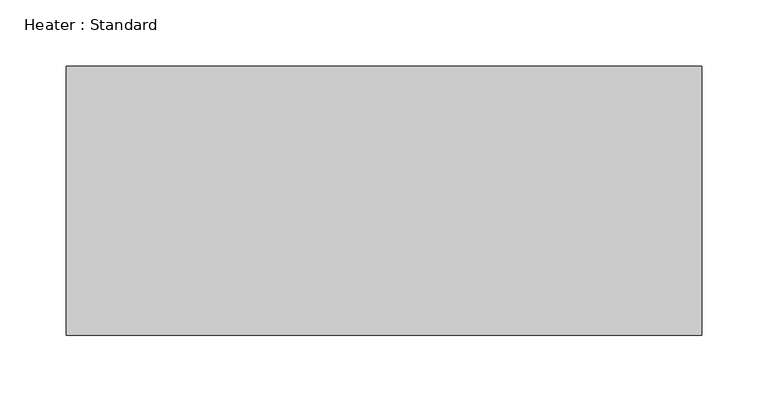
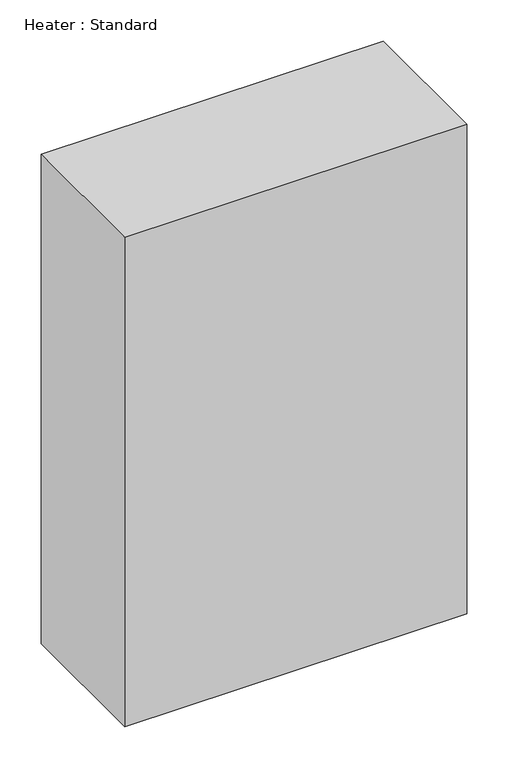
"""IFC4 building model written with IfcOpenShell, lengths in millimetres: proxy geometry, Heater : Standard."""

import ifcopenshell
import ifcopenshell.guid

model = None  # the IFC model being written
_history = None  # IfcOwnerHistory: only IFC2X3 demands one
_inside = {}  # id of a spatial element -> (the spatial element, [elements in it])
_under = {}  # id of a project, library or spatial element -> (it, [spatial elements below it])
_declared = {}  # id of a project -> (the project, [libraries it declares])
_typed = {}  # id of a type object -> (the type object, [elements of that type])
_made_of = {}  # id of a material, layer set ... -> (it, [elements and type objects made of it])


def new_model(schema):
    """Start an empty IFC model of exactly this schema.

    Asked for "IFC4X3", IfcOpenShell would pick the latest addendum, in which some entities
    have other attributes; the version numbers below select the first issue.
    IFC2X3 requires an IfcOwnerHistory on every rooted entity: one is made here for all.
    """
    global model, _history
    if schema == "IFC4X3":
        model = ifcopenshell.file(schema_version=(4, 3, 0, 0))
    else:
        model = ifcopenshell.file(schema=schema)
    _inside.clear()
    _under.clear()
    _declared.clear()
    _typed.clear()
    _made_of.clear()
    _history = None
    if model.schema == "IFC2X3":
        org = make("IfcOrganization", Name="unknown")
        user = make(
            "IfcPersonAndOrganization",
            ThePerson=make("IfcPerson", FamilyName="unknown"),
            TheOrganization=org,
        )
        app = make(
            "IfcApplication",
            ApplicationDeveloper=org,
            Version="unknown",
            ApplicationFullName="unknown",
            ApplicationIdentifier="unknown",
        )
        _history = make(
            "IfcOwnerHistory",
            OwningUser=user,
            OwningApplication=app,
            ChangeAction="ADDED",
            CreationDate=0,
        )
    return model


def make(cls, **values):
    """One entity of the class cls with the attributes given. An attribute that is None is left unset."""
    return model.create_entity(
        cls, **{name: value for name, value in values.items() if value is not None}
    )


def rooted(cls, **values):
    """An entity with a GlobalId (a new one), such as an element, a storey or a relation."""
    return make(cls, GlobalId=ifcopenshell.guid.new(), OwnerHistory=_history, **values)


def si_unit(unit_type, name, prefix=None):
    """IfcSIUnit, for example si_unit("LENGTHUNIT", "METRE", prefix="MILLI")."""
    return make("IfcSIUnit", UnitType=unit_type, Prefix=prefix, Name=name)


def assignment(units):
    """IfcUnitAssignment: the units of a project."""
    return None if units is None else make("IfcUnitAssignment", Units=units)


def point(xyz):
    """IfcCartesianPoint."""
    return None if xyz is None else make("IfcCartesianPoint", Coordinates=xyz)


def direction(xyz):
    """IfcDirection."""
    return None if xyz is None else make("IfcDirection", DirectionRatios=xyz)


def frame(location, z_axis=None, x_axis=None):
    """IfcAxis2Placement3D, a coordinate frame: its origin and axes. An axis left out is left unset."""
    return make(
        "IfcAxis2Placement3D",
        Location=point(location),
        Axis=direction(z_axis),
        RefDirection=direction(x_axis),
    )


def origin():
    """The frame at (0, 0, 0) with its axes left unset."""
    return frame((0.0, 0.0, 0.0))


def origin_with_axes():
    """The frame at (0, 0, 0) with the z axis (0, 0, 1) and the x axis (1, 0, 0) written out."""
    return frame((0.0, 0.0, 0.0), z_axis=(0.0, 0.0, 1.0), x_axis=(1.0, 0.0, 0.0))


def place(relative_to, where):
    """IfcLocalPlacement: puts the frame where relative to a parent placement (None: the world)."""
    return make(
        "IfcLocalPlacement", PlacementRelTo=relative_to, RelativePlacement=where
    )


def context(
    kind, dimensions, precision=None, world=None, true_north=None, identifier=None
):
    """IfcGeometricRepresentationContext, for example the 3D "Model" context."""
    return make(
        "IfcGeometricRepresentationContext",
        ContextIdentifier=identifier,
        ContextType=kind,
        CoordinateSpaceDimension=dimensions,
        Precision=precision,
        WorldCoordinateSystem=world,
        TrueNorth=true_north,
    )


def project(units=None, contexts=None):
    """IfcProject with its units and contexts."""
    return rooted(
        "IfcProject",
        Name="project",
        RepresentationContexts=contexts,
        UnitsInContext=assignment(units),
    )


def spatial(cls, under=None, at=None, **own):
    """A site, building, storey or space (cls), placed at a placement, below another one or the project."""
    s = rooted(cls, ObjectPlacement=at, **own)
    if under is not None:
        _under.setdefault(under.id(), (under, []))[1].append(s)
    return s


def polyline(points):
    """IfcPolyline through the points."""
    return make("IfcPolyline", Points=[point(p) for p in points])


def outline(outer, holes=None, kind="AREA"):
    """IfcArbitraryClosedProfileDef: a profile drawn as a closed curve; with holes, ...WithVoids."""
    if holes is None:
        return make("IfcArbitraryClosedProfileDef", ProfileType=kind, OuterCurve=outer)
    return make(
        "IfcArbitraryProfileDefWithVoids",
        ProfileType=kind,
        OuterCurve=outer,
        InnerCurves=holes,
    )


def extrude(swept, where, along, depth):
    """IfcExtrudedAreaSolid: the profile swept, set in the frame where, extruded along a direction by depth."""
    return make(
        "IfcExtrudedAreaSolid",
        SweptArea=swept,
        Position=where,
        ExtrudedDirection=direction(along),
        Depth=depth,
    )


def shape(context_of_items, identifier, shape_type, items):
    """IfcShapeRepresentation: the items that make up one representation, for example the "Body"."""
    return make(
        "IfcShapeRepresentation",
        ContextOfItems=context_of_items,
        RepresentationIdentifier=identifier,
        RepresentationType=shape_type,
        Items=items,
    )


def source(mapping_origin, context_of_items, identifier, shape_type, items):
    """IfcRepresentationMap: a shape defined once, which mapped items show again and again."""
    return make(
        "IfcRepresentationMap",
        MappingOrigin=mapping_origin,
        MappedRepresentation=shape(context_of_items, identifier, shape_type, items),
    )


def transform(
    local_origin,
    x_axis=None,
    y_axis=None,
    z_axis=None,
    scale=None,
    scale2=None,
    scale3=None,
    uniform=True,
):
    """IfcCartesianTransformationOperator3D, or its non-uniform kind. x_axis, y_axis, z_axis: its Axis1, 2, 3."""
    if uniform:
        return make(
            "IfcCartesianTransformationOperator3D",
            Axis1=direction(x_axis),
            Axis2=direction(y_axis),
            LocalOrigin=point(local_origin),
            Scale=scale,
            Axis3=direction(z_axis),
        )
    return make(
        "IfcCartesianTransformationOperator3DnonUniform",
        Axis1=direction(x_axis),
        Axis2=direction(y_axis),
        LocalOrigin=point(local_origin),
        Scale=scale,
        Axis3=direction(z_axis),
        Scale2=scale2,
        Scale3=scale3,
    )


def mapped(mapping_source, mapping_target):
    """IfcMappedItem: shows the shape of a source again, moved by a transform."""
    return make(
        "IfcMappedItem", MappingSource=mapping_source, MappingTarget=mapping_target
    )


def made_of(thing, what):
    """Note that an element or type object is made of a material, layer set ...; save() writes the relation."""
    if what is not None:
        _made_of.setdefault(what.id(), (what, []))[1].append(thing)
    return thing


def element(
    cls,
    number,
    at=None,
    inside=None,
    cuts=None,
    type_object=None,
    material=None,
    context=None,
    identifier="Body",
    shape_type=None,
    held_by="IfcProductDefinitionShape",
    body=None,
    shapes=None,
    **own,
):
    """One element of the class cls, such as IfcWall. Its Tag is "e" and its number.

    at: its placement. inside: the storey or other place that contains it. cuts: it is an
    opening in that element (IfcRelVoidsElement). A single representation is given by context,
    identifier, shape_type and body (its items); several are given by shapes. held_by: the class
    of the entity that holds the representations. save() writes the other relations.
    """
    e = rooted(cls, Tag="e%d" % number, ObjectPlacement=at, **own)
    if body is not None:
        shapes = [shape(context, identifier, shape_type, body)]
    if shapes is not None:
        e.Representation = make(held_by, Representations=shapes)
    if inside is not None:
        _inside.setdefault(inside.id(), (inside, []))[1].append(e)
    if cuts is not None:
        rooted(
            "IfcRelVoidsElement", RelatingBuildingElement=cuts, RelatedOpeningElement=e
        )
    if type_object is not None:
        _typed.setdefault(type_object.id(), (type_object, []))[1].append(e)
    return made_of(e, material)


def aggregate(whole, parts):
    """IfcRelAggregates: a whole, such as a stair, and the parts it consists of."""
    return rooted("IfcRelAggregates", RelatingObject=whole, RelatedObjects=parts)


def save(model, path):
    """Write the relations noted so far, then the file.

    IfcRelAggregates (storeys below a building ...), IfcRelContainedInSpatialStructure (elements
    in a storey), IfcRelDefinesByType, IfcRelAssociatesMaterial and IfcRelDeclares: one each for
    every whole, place, type object, material and project.
    """
    for whole, parts in _under.values():
        aggregate(whole, parts)
    for where, things in _inside.values():
        rooted(
            "IfcRelContainedInSpatialStructure",
            RelatedElements=things,
            RelatingStructure=where,
        )
    for kind, things in _typed.values():
        rooted("IfcRelDefinesByType", RelatedObjects=things, RelatingType=kind)
    for what, things in _made_of.values():
        rooted("IfcRelAssociatesMaterial", RelatedObjects=things, RelatingMaterial=what)
    for by, libraries in _declared.values():
        rooted("IfcRelDeclares", RelatingContext=by, RelatedDefinitions=libraries)
    model.write(path)


def heater_standard_9b13520e(model_context):
    return source(origin(), model_context, "Body", "SweptSolid", [
        extrude(outline(polyline([(240.0101563, 0.0), (240.0101563, -203.2), (-240.0101562, -203.2), (-240.0101562, 0.0), (240.0101563, 0.0)])), origin_with_axes(), (0.0, 0.0, 1.0), 726.4796875),
    ])


if __name__ == "__main__":
    model = new_model("IFC4")
    model_context = context("Model", 3, world=origin())
    ifc_project = project(units=[si_unit("LENGTHUNIT", "METRE", prefix="MILLI")], contexts=[model_context])
    site = spatial("IfcSite", under=ifc_project)
    building = spatial("IfcBuilding", under=site)
    placement = place(None, origin())
    heater_standard_shape = heater_standard_9b13520e(model_context)
    element("IfcBuildingElementProxy", 1, Name="Heater : Standard", ObjectType="Heater : Standard", at=placement, inside=building, context=model_context, shape_type="MappedRepresentation", body=[
        mapped(heater_standard_shape, transform((0.0, 0.0, 0.0), x_axis=(1.0, 0.0, 0.0), y_axis=(0.0, 1.0, 0.0), z_axis=(0.0, 0.0, 1.0))),
    ])
    save(model, "model.ifc")

# Revit data of these elements
# Type "Heater : Standard"
#   Label = "H"
#   Width = 0' - 8"
#   Voltage = 120 V
#   Length = 1' - 6 115/128"
#   Height = 2' - 4 77/128"
#   Apparent Load = 1500 VA
#   Number of Poles = 1
#   Load Classification = Heating
#   Heater Material = none
#   Default Elevation = 0
